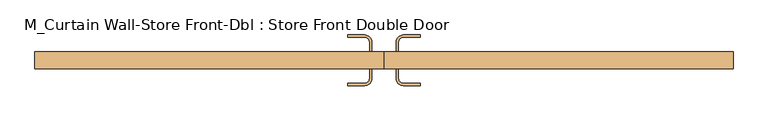
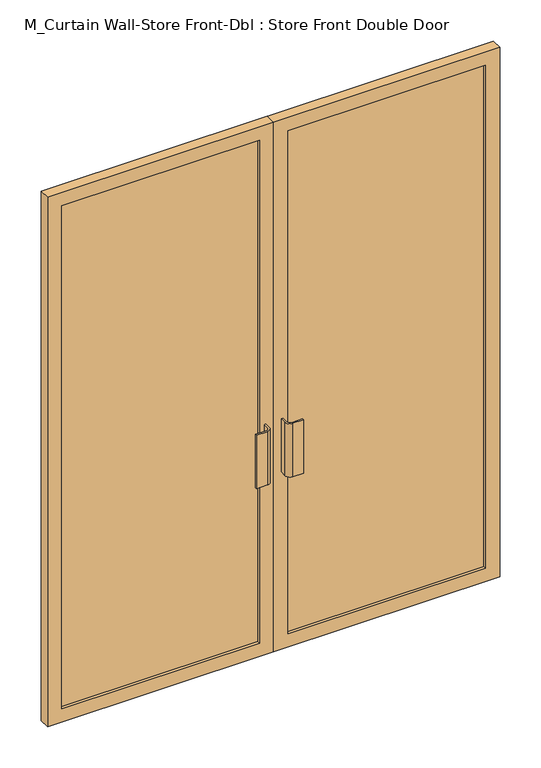
"""IFC4 building model written with IfcOpenShell, lengths in millimetres: door geometry, M_Curtain Wall-Store Front-Dbl : Store Front Double Door."""

from ifc_helpers import new_model, si_unit, point, frame, frame_2d, origin, place, context, project, spatial, polyline, circle_curve, trimmed, segment, composite_curve, outline, extrude, source, transform, mapped, element, save


def m_curtain_wall_store_front_dbl_store_front_double_door_b335b37c(model_context):
    return source(origin(), model_context, "Body", "SweptSolid", [
        extrude(outline(composite_curve([segment(trimmed(circle_curve(frame_2d((-50.8, -14.85)), 19.05), [point((-31.75, -14.85))], [point((-50.8, -33.9))], False, "CARTESIAN"), True, "CONTINUOUS"), segment(polyline([(-50.8, -33.9), (-95.25, -33.9), (-95.25, -27.55), (-50.8, -27.55)]), True, "CONTINUOUS"), segment(trimmed(circle_curve(frame_2d((-50.8, -14.85)), 12.7), [point((-50.8, -27.55))], [point((-38.1, -14.85))], True, "CARTESIAN"), True, "CONTINUOUS"), segment(polyline([(-38.1, -14.85), (-38.1, 10.55), (-31.75, 10.55), (-31.75, -14.85)]), True, "CONTINUOUS")], self_intersect=False)), frame((0.0, 0.0, 762.0), z_axis=(0.0, 0.0, 1.0), x_axis=(1.0, 0.0, 0.0)), (0.0, 0.0, 1.0), 228.6),
        extrude(outline(composite_curve([segment(polyline([(31.75, -14.85), (31.75, 10.55), (38.1, 10.55), (38.1, -14.85)]), True, "CONTINUOUS"), segment(trimmed(circle_curve(frame_2d((50.8, -14.85)), 12.7), [point((38.1, -14.85))], [point((50.8, -27.55))], True, "CARTESIAN"), True, "CONTINUOUS"), segment(polyline([(50.8, -27.55), (95.25, -27.55), (95.25, -33.9), (50.8, -33.9)]), True, "CONTINUOUS"), segment(trimmed(circle_curve(frame_2d((50.8, -14.85)), 19.05), [point((50.8, -33.9))], [point((31.75, -14.85))], False, "CARTESIAN"), True, "CONTINUOUS")], self_intersect=False)), frame((0.0, 0.0, 762.0), z_axis=(0.0, 0.0, 1.0), x_axis=(1.0, 0.0, 0.0)), (0.0, 0.0, 1.0), 228.6),
        extrude(outline(composite_curve([segment(polyline([(-31.75, 80.4), (-31.75, 55.0), (-38.1, 55.0), (-38.1, 80.4)]), True, "CONTINUOUS"), segment(trimmed(circle_curve(frame_2d((-50.8, 80.4)), 12.7), [point((-38.1, 80.4))], [point((-50.8, 93.1))], True, "CARTESIAN"), True, "CONTINUOUS"), segment(polyline([(-50.8, 93.1), (-95.25, 93.1), (-95.25, 99.45), (-50.8, 99.45)]), True, "CONTINUOUS"), segment(trimmed(circle_curve(frame_2d((-50.8, 80.4)), 19.05), [point((-50.8, 99.45))], [point((-31.75, 80.4))], False, "CARTESIAN"), True, "CONTINUOUS")], self_intersect=False)), frame((0.0, 0.0, 762.0), z_axis=(0.0, 0.0, 1.0), x_axis=(1.0, 0.0, 0.0)), (0.0, 0.0, 1.0), 228.6),
        extrude(outline(composite_curve([segment(trimmed(circle_curve(frame_2d((50.8, 80.4)), 19.05), [point((31.75, 80.4))], [point((50.8, 99.45))], False, "CARTESIAN"), True, "CONTINUOUS"), segment(polyline([(50.8, 99.45), (95.25, 99.45), (95.25, 93.1), (50.8, 93.1)]), True, "CONTINUOUS"), segment(trimmed(circle_curve(frame_2d((50.8, 80.4)), 12.7), [point((50.8, 93.1))], [point((38.1, 80.4))], True, "CARTESIAN"), True, "CONTINUOUS"), segment(polyline([(38.1, 80.4), (38.1, 55.0), (31.75, 55.0), (31.75, 80.4)]), True, "CONTINUOUS")], self_intersect=False)), frame((0.0, 0.0, 762.0), z_axis=(0.0, 0.0, 1.0), x_axis=(1.0, 0.0, 0.0)), (0.0, 0.0, 1.0), 228.6),
        extrude(outline(polyline([(862.2944444, 23.25), (57.94375, 23.25), (57.94375, 42.3), (862.2944444, 42.3), (862.2944444, 23.25)])), frame((0.0, 0.0, 57.15), z_axis=(0.0, 0.0, 1.0), x_axis=(1.0, 0.0, 0.0)), (0.0, 0.0, 1.0), 2160.7),
        extrude(outline(polyline([(-57.94375, 23.25), (-862.2944444, 23.25), (-862.2944444, 42.3), (-57.94375, 42.3), (-57.94375, 23.25)])), frame((0.0, 0.0, 57.15), z_axis=(0.0, 0.0, 1.0), x_axis=(1.0, 0.0, 0.0)), (0.0, 0.0, 1.0), 2160.7),
        extrude(outline(polyline([(2275.0, 0.79375), (0.0, 0.79375), (0.0, 919.4444444), (2275.0, 919.4444444), (2275.0, 0.79375)]), holes=[polyline([(2217.85, 57.94375), (2217.85, 862.2944444), (57.15, 862.2944444), (57.15, 57.94375), (2217.85, 57.94375)])]), frame((0.0, 10.55, 0.0), z_axis=(0.0, 1.0, 0.0), x_axis=(0.0, 0.0, 1.0)), (0.0, 0.0, 1.0), 44.45),
        extrude(outline(polyline([(2275.0, -0.79375), (2275.0, -919.4444444), (0.0, -919.4444444), (0.0, -0.79375), (2275.0, -0.79375)]), holes=[polyline([(2217.85, -862.2944444), (2217.85, -57.94375), (57.15, -57.94375), (57.15, -862.2944444), (2217.85, -862.2944444)])]), frame((0.0, 10.55, 0.0), z_axis=(0.0, 1.0, 0.0), x_axis=(0.0, 0.0, 1.0)), (0.0, 0.0, 1.0), 44.45),
    ])


if __name__ == "__main__":
    model = new_model("IFC4")
    model_context = context("Model", 3, world=origin())
    ifc_project = project(units=[si_unit("LENGTHUNIT", "METRE", prefix="MILLI")], contexts=[model_context])
    site = spatial("IfcSite", under=ifc_project)
    building = spatial("IfcBuilding", under=site)
    placement = place(None, origin())
    m_curtain_wall_store_front_dbl_store_front_double_door_shape = m_curtain_wall_store_front_dbl_store_front_double_door_b335b37c(model_context)
    element("IfcDoor", 1, ObjectType="M_Curtain Wall-Store Front-Dbl : Store Front Double Door", at=placement, inside=building, context=model_context, shape_type="MappedRepresentation", body=[
        mapped(m_curtain_wall_store_front_dbl_store_front_double_door_shape, transform((0.0, 0.0, 0.0), x_axis=(1.0, 0.0, 0.0), y_axis=(0.0, 1.0, 0.0), z_axis=(0.0, 0.0, 1.0))),
    ])
    save(model, "model.ifc")

# Revit data of these elements
# Type "M_Curtain Wall-Store Front-Dbl : Store Front Double Door"
#   Type Mark = "34"
#   Offset = 0.055 m
#   Function = 1
#   Define Thermal Properties by = 1
#   Material = Metal - Aluminum
#   Glazing Material = Window - Glass
#   Assembly Code = ""
# Element 1 (IfcDoor, "M_Curtain Wall-Store Front-Dbl : Store Front Double Door")
#   Materials on its faces: "Metal - Aluminum", "Window - Glass"
# Materials
#   "Metal - Aluminum": class "Unassigned", colour RGB 247 247 247, transparency 0, Comments = "Rendering appearance not upgraded "
#   "Window - Glass": class "Glas", colour RGB 128 128 255, transparency 0.75
